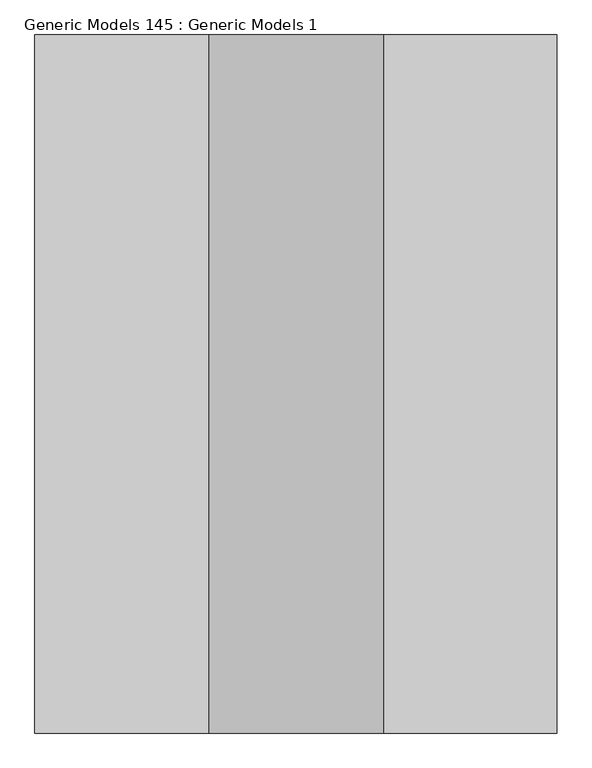
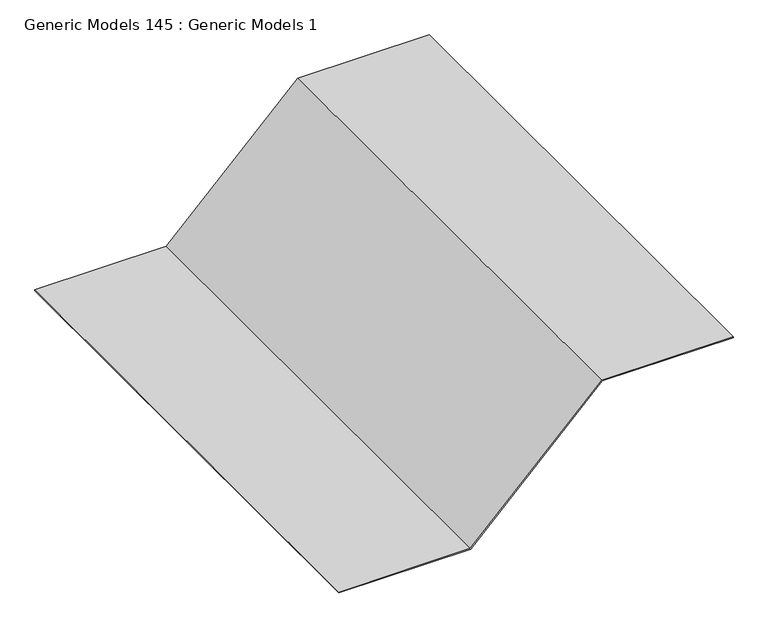
"""IFC4 building model written with IfcOpenShell, lengths in millimetres: proxy geometry, Generic Models 145 : Generic Models 1."""

from ifc_helpers import new_model, si_unit, frame, origin, place, context, project, spatial, polyline, outline, extrude, source, transform, mapped, element, save


def generic_models_145_generic_models_1_d1ee8326(model_context):
    return source(origin(), model_context, "Body", "SweptSolid", [
        extrude(outline(polyline([(-155.575, 52785.9625), (-153.9875, 52785.9625), (-153.9875, 52482.353125), (-458.7875, 52177.553125), (-458.7875, 51873.410689), (-460.375, 51873.410689), (-460.375, 52178.210689), (-155.575, 52483.010689), (-155.575, 52785.9625)])), frame((0.0, 0.0, 0.0), z_axis=(0.0, 1.0, 0.0), x_axis=(0.0, 0.0, 1.0)), (0.0, 0.0, 1.0), 1219.2),
    ])


if __name__ == "__main__":
    model = new_model("IFC4")
    model_context = context("Model", 3, world=origin())
    ifc_project = project(units=[si_unit("LENGTHUNIT", "METRE", prefix="MILLI")], contexts=[model_context])
    site = spatial("IfcSite", under=ifc_project)
    building = spatial("IfcBuilding", under=site)
    placement = place(None, origin())
    generic_models_145_generic_models_1_shape = generic_models_145_generic_models_1_d1ee8326(model_context)
    element("IfcBuildingElementProxy", 1, Name="Generic Models 145 : Generic Models 1", ObjectType="Generic Models 145 : Generic Models 1", at=placement, inside=building, context=model_context, shape_type="MappedRepresentation", body=[
        mapped(generic_models_145_generic_models_1_shape, transform((0.0, 0.0, 0.0), x_axis=(1.0, 0.0, 0.0), y_axis=(0.0, 1.0, 0.0), z_axis=(0.0, 0.0, 1.0))),
    ])
    save(model, "model.ifc")

# Revit data of these elements
# Element 1 (IfcBuildingElementProxy, "Generic Models 145 : Generic Models 1")
#   Materials on its faces: "6 MIL VAPOR BARRIER"
# Materials
#   "6 MIL VAPOR BARRIER": class "Generic", colour RGB 66 158 52, transparency 0, Cost = 0
